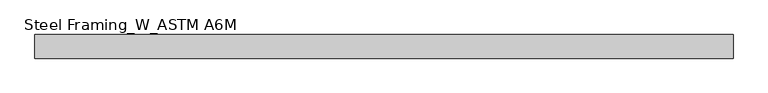
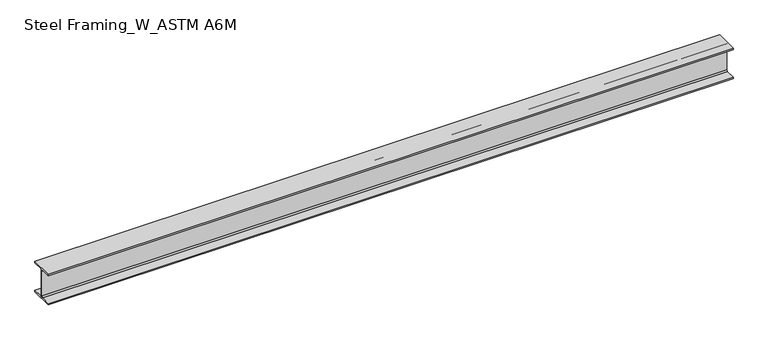
"""IFC4 building model written with IfcOpenShell, lengths in millimetres: beam geometry, Steel Framing_W_ASTM A6M : H_SB_AR_S02_W360x91_G2."""

from ifc_helpers import new_model, si_unit, point, frame, frame_2d, origin, place, context, project, spatial, polyline, circle_curve, trimmed, segment, composite_curve, outline, extrude, source, transform, mapped, element, save


def steel_framing_w_astm_a6m_6b956c3c(model_context):
    return source(origin(), model_context, "Body", "SweptSolid", [
        extrude(outline(composite_curve([segment(polyline([(127.0, -160.1), (127.0, -176.5), (-127.0, -176.5), (-127.0, -160.1), (-19.865, -160.1)]), True, "CONTINUOUS"), segment(trimmed(circle_curve(frame_2d((-19.865, -145.0)), 15.1), [point((-19.865, -160.1))], [point((-4.765, -145.0))], True, "CARTESIAN"), True, "CONTINUOUS"), segment(polyline([(-4.765, -145.0), (-4.765, 145.0)]), True, "CONTINUOUS"), segment(trimmed(circle_curve(frame_2d((-19.865, 145.0)), 15.1), [point((-4.765, 145.0))], [point((-19.865, 160.1))], True, "CARTESIAN"), True, "CONTINUOUS"), segment(polyline([(-19.865, 160.1), (-127.0, 160.1), (-127.0, 176.5), (127.0, 176.5), (127.0, 160.1), (19.865, 160.1)]), True, "CONTINUOUS"), segment(trimmed(circle_curve(frame_2d((19.865, 145.0)), 15.1), [point((19.865, 160.1))], [point((4.765, 145.0))], True, "CARTESIAN"), True, "CONTINUOUS"), segment(polyline([(4.765, 145.0), (4.765, -145.0)]), True, "CONTINUOUS"), segment(trimmed(circle_curve(frame_2d((19.865, -145.0)), 15.1), [point((4.765, -145.0))], [point((19.865, -160.1))], True, "CARTESIAN"), True, "CONTINUOUS"), segment(polyline([(19.865, -160.1), (127.0, -160.1)]), True, "CONTINUOUS")], self_intersect=False)), frame((-3753.7, 0.0, 0.0), z_axis=(1.0, 0.0, 0.0), x_axis=(0.0, 1.0, 0.0)), (0.0, 0.0, 1.0), 7507.4),
    ])


if __name__ == "__main__":
    model = new_model("IFC4")
    model_context = context("Model", 3, world=origin())
    ifc_project = project(units=[si_unit("LENGTHUNIT", "METRE", prefix="MILLI")], contexts=[model_context])
    site = spatial("IfcSite", under=ifc_project)
    building = spatial("IfcBuilding", under=site)
    placement = place(None, origin())
    steel_framing_w_astm_a6m_shape = steel_framing_w_astm_a6m_6b956c3c(model_context)
    element("IfcBeam", 1, ObjectType="Steel Framing_W_ASTM A6M : H_SB_AR_S02_W360x91_G2", at=placement, inside=building, context=model_context, shape_type="MappedRepresentation", body=[
        mapped(steel_framing_w_astm_a6m_shape, transform((0.0, 0.0, 0.0), x_axis=(1.0, 0.0, 0.0), y_axis=(0.0, 1.0, 0.0), z_axis=(0.0, 0.0, 1.0))),
    ])
    save(model, "model.ifc")

# Revit data of these elements
# Type "Steel Framing_W_ASTM A6M : H_SB_AR_S02_W360x91_G2"
#   Type Mark = "G2"
#   Section Name Key = "W14x61"
#   Width = 25.4 cm
#   Web Thickness = 0.953 cm
#   Web Fillet = 1.51 cm
#   Warping Constant = 1260000.0 cm⁶
#   Torsional Moment of Inertia = 91.20 cm⁴
#   Section Area = 115.0 cm²
#   Plastic Modulus weak axis = 537.0 cm³
#   Plastic Modulus strong axis = 1670.0 cm³
#   Perimeter = 1.68 m²/m
#   Nominal Weight = 91.00 kgf/m
#   Moment of Inertia weak axis = 4450.00 cm⁴
#   Moment of Inertia strong axis = 26600.00 cm⁴
#   Height = 35.3 cm
#   Flange Thickness = 1.64 cm
#   Elastic Modulus weak axis = 352.0 cm³
#   Elastic Modulus strong axis = 1510.0 cm³
#   Centroid Vertical = 17.65 cm
#   Centroid Horizontal = 12.7 cm
#   Length [instance default] = 1500 mm
#   Structural Material [instance default] = Steel, 45-345
#   Bolt Spacing = 0
#   Assembly Code = ""
# Element 1 (IfcBeam, "Steel Framing_W_ASTM A6M : H_SB_AR_S02_W360x91_G2")
#   Materials on its faces: "Steel, 45-345"
# Materials
#   "Steel, 45-345": class "Metal", colour RGB 189 187 185, transparency 0, Description = "Steel 345 MPa", Cost = 0
